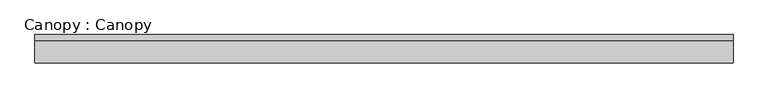
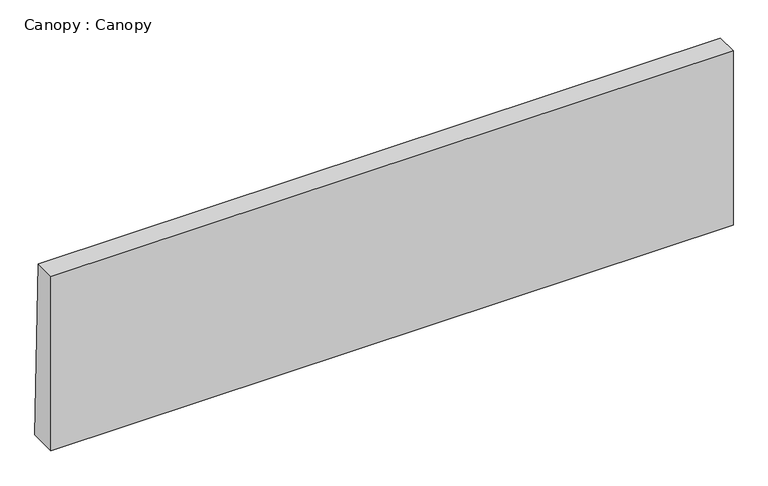
"""IFC4 building model written with IfcOpenShell, lengths in millimetres: proxy geometry, Canopy : Canopy."""

from ifc_helpers import new_model, si_unit, frame, origin, place, context, project, spatial, polyline, outline, extrude, source, transform, mapped, element, save


def canopy_canopy_da837555(model_context):
    return source(origin(), model_context, "Body", "SweptSolid", [
        extrude(outline(polyline([(150.0, 0.0), (0.0, 0.0), (0.0, 1000.0), (120.0, 1000.0), (150.0, 0.0)])), frame((-1850.0, 0.0, 0.0), z_axis=(1.0, 0.0, 0.0), x_axis=(0.0, 1.0, 0.0)), (0.0, 0.0, 1.0), 3700.0),
    ])


if __name__ == "__main__":
    model = new_model("IFC4")
    model_context = context("Model", 3, world=origin())
    ifc_project = project(units=[si_unit("LENGTHUNIT", "METRE", prefix="MILLI")], contexts=[model_context])
    site = spatial("IfcSite", under=ifc_project)
    building = spatial("IfcBuilding", under=site)
    placement = place(None, origin())
    canopy_canopy_shape = canopy_canopy_da837555(model_context)
    element("IfcBuildingElementProxy", 1, Name="Canopy : Canopy", ObjectType="Canopy : Canopy", at=placement, inside=building, context=model_context, shape_type="MappedRepresentation", body=[
        mapped(canopy_canopy_shape, transform((0.0, 0.0, 0.0), x_axis=(1.0, 0.0, 0.0), y_axis=(0.0, 1.0, 0.0), z_axis=(0.0, 0.0, 1.0))),
    ])
    save(model, "model.ifc")

# Revit data of these elements
# Type "Canopy : Canopy"
#   Type Comments = "CV-AG"
#   H_Rebar Ratio = 0.1
#   Canopy Width [instance default] = 1700 mm
#   Canopy Length [instance default] = 1000 mm
#   Canopy L.P = 120 mm
#   Canopy H.P = 150 mm
#   구조재료 = Concrete_f'c=28MPa(Cylender)
#   Default Elevation = 0
# Element 1 (IfcBuildingElementProxy, "Canopy : Canopy")
#   Canopy Width = 3700 mm
#   Materials on its faces: "Concrete_f'c=28MPa(Cylender)"
# Materials
#   "Concrete_f'c=28MPa(Cylender)": class "Concrete", colour RGB 176 176 176, transparency 0, Description = "Reinf. Conc.", Cost = 0, Image = Concrete.Cast-In-Place.Flat.Polished.Grey.jpg
